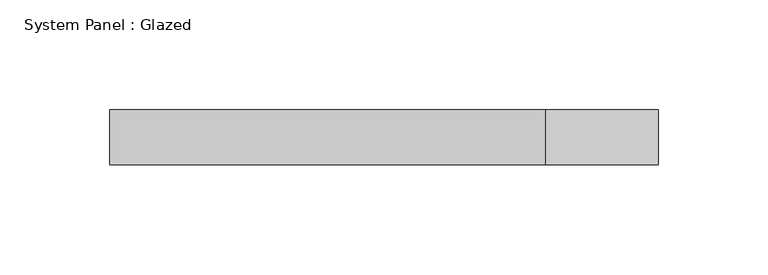
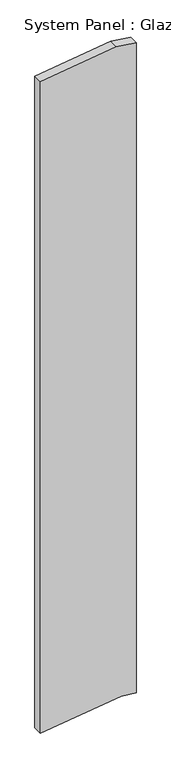
"""IFC4 building model written with IfcOpenShell, lengths in millimetres: plate geometry, System Panel : Glazed."""

from ifc_helpers import new_model, si_unit, frame, origin, place, context, project, spatial, polyline, outline, extrude, source, transform, mapped, element, save


def system_panel_glazed_c840bec2(model_context):
    return source(origin(), model_context, "Body", "SweptSolid", [
        extrude(outline(polyline([(0.0, -125.0), (28.4114608, 85.6318823), (23.8703754, 125.0), (1820.8662712, 125.0), (1826.7926752, 73.6237549), (1800.0009018, -125.0), (0.0, -125.0)])), frame((0.0, -49.5, 0.0), z_axis=(0.0, 1.0, 0.0), x_axis=(0.0, 0.0, 1.0)), (0.0, 0.0, 1.0), 25.0),
    ])


if __name__ == "__main__":
    model = new_model("IFC4")
    model_context = context("Model", 3, world=origin())
    ifc_project = project(units=[si_unit("LENGTHUNIT", "METRE", prefix="MILLI")], contexts=[model_context])
    site = spatial("IfcSite", under=ifc_project)
    building = spatial("IfcBuilding", under=site)
    placement = place(None, origin())
    system_panel_glazed_shape = system_panel_glazed_c840bec2(model_context)
    element("IfcPlate", 1, ObjectType="System Panel : Glazed", at=placement, inside=building, context=model_context, shape_type="MappedRepresentation", body=[
        mapped(system_panel_glazed_shape, transform((0.0, 0.0, 0.0), x_axis=(1.0, 0.0, 0.0), y_axis=(0.0, 1.0, 0.0), z_axis=(0.0, 0.0, 1.0))),
    ])
    save(model, "model.ifc")

# Revit data of these elements
# Element 1 (IfcPlate, "System Panel : Glazed")
#   Materials on its faces: "Glass"
# Materials
#   "Glass": class "Glass", colour RGB 218 227 224, transparency 0.85, Description = "Soda Lime Glass", Cost = 0
